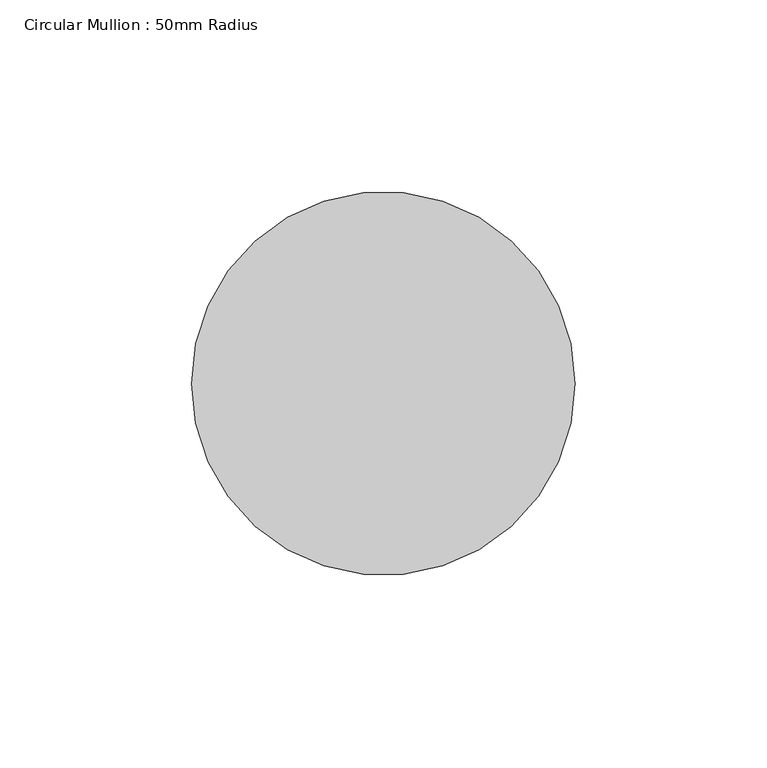
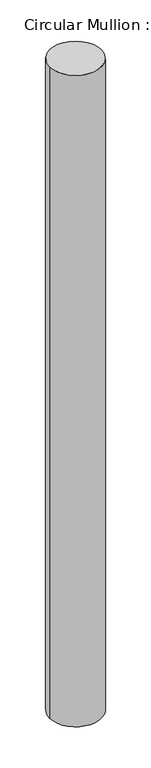
"""IFC4 building model written with IfcOpenShell, lengths in millimetres: member geometry, Circular Mullion : 50mm Radius."""

from ifc_helpers import new_model, si_unit, point, frame, origin, origin_2d, place, context, project, spatial, circle_curve, trimmed, segment, composite_curve, outline, extrude, source, transform, mapped, element, save


def circular_mullion_50mm_radius_fde642d1(model_context):
    return source(origin(), model_context, "Body", "SweptSolid", [
        extrude(outline(composite_curve([segment(trimmed(circle_curve(origin_2d(), 50.0), [point((50.0, 0.0))], [point((-50.0, 0.0))], False, "CARTESIAN"), True, "CONTINUOUS"), segment(trimmed(circle_curve(origin_2d(), 50.0), [point((-50.0, 0.0))], [point((50.0, 0.0))], False, "CARTESIAN"), True, "CONTINUOUS")], self_intersect=False)), frame((0.0, 0.0, -1331.2304132), z_axis=(0.0, 0.0, 1.0), x_axis=(1.0, 0.0, 0.0)), (0.0, 0.0, 1.0), 1331.2304132),
    ])


if __name__ == "__main__":
    model = new_model("IFC4")
    model_context = context("Model", 3, world=origin())
    ifc_project = project(units=[si_unit("LENGTHUNIT", "METRE", prefix="MILLI")], contexts=[model_context])
    site = spatial("IfcSite", under=ifc_project)
    building = spatial("IfcBuilding", under=site)
    placement = place(None, origin())
    circular_mullion_50mm_radius_shape = circular_mullion_50mm_radius_fde642d1(model_context)
    element("IfcMember", 1, ObjectType="Circular Mullion : 50mm Radius", at=placement, inside=building, context=model_context, shape_type="MappedRepresentation", body=[
        mapped(circular_mullion_50mm_radius_shape, transform((0.0, 0.0, 0.0), x_axis=(1.0, 0.0, 0.0), y_axis=(0.0, 1.0, 0.0), z_axis=(0.0, 0.0, 1.0))),
    ])
    save(model, "model.ifc")

# Revit data of these elements
# Type "Circular Mullion : 50mm Radius"
#   built-in parameter 1007350 = 0.164042 (stored number, unit not read)
# Element 1 (IfcMember, "Circular Mullion : 50mm Radius")
#   Materials on its faces: "Aluminium"
# Materials
#   "Aluminium": class "Metal", colour RGB 247 247 247, transparency 0, Description = "Aluminium 6061", Cost = 0
